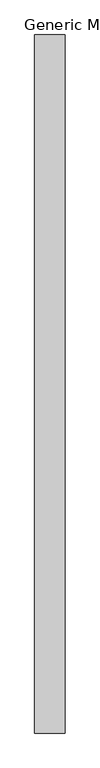
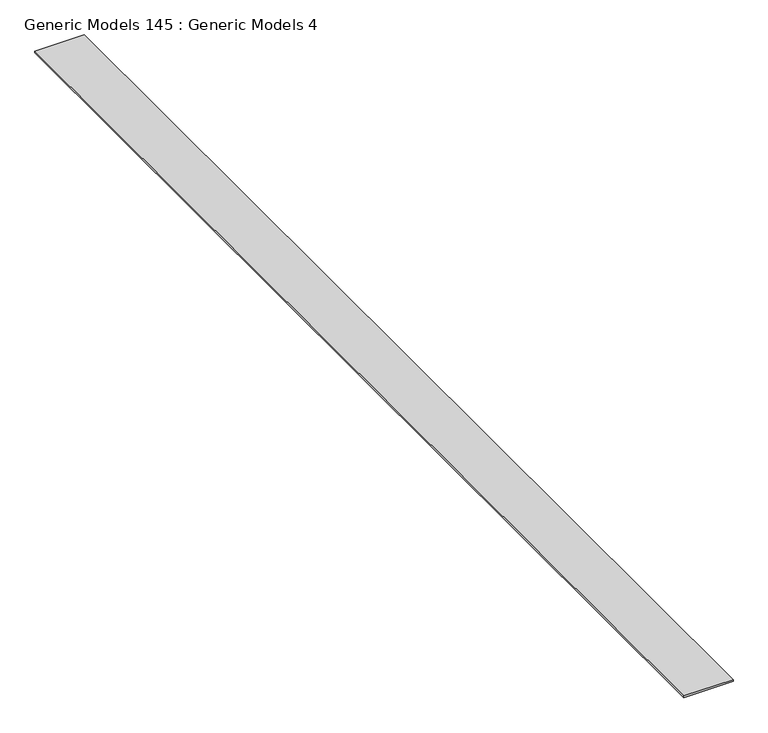
"""IFC4 building model written with IfcOpenShell, lengths in millimetres: proxy geometry, Generic Models 145 : Generic Models 4."""

from ifc_helpers import new_model, si_unit, frame, origin, place, context, project, spatial, polyline, outline, extrude, source, transform, mapped, element, save


def generic_models_145_generic_models_4_5156f356(model_context):
    return source(origin(), model_context, "Body", "SweptSolid", [
        extrude(outline(polyline([(-5950.1236296, -5493.3230338), (-6498.6122941, -5493.3230338), (-6498.6122941, 7054.2769662), (-5950.1236296, 7054.2769662), (-5950.1236296, -5493.3230338)])), frame((0.0, 0.0, 123278.646), z_axis=(0.0, 0.0, 1.0), x_axis=(1.0, 0.0, 0.0)), (0.0, 0.0, 1.0), 19.05),
    ])


if __name__ == "__main__":
    model = new_model("IFC4")
    model_context = context("Model", 3, world=origin())
    ifc_project = project(units=[si_unit("LENGTHUNIT", "METRE", prefix="MILLI")], contexts=[model_context])
    site = spatial("IfcSite", under=ifc_project)
    building = spatial("IfcBuilding", under=site)
    placement = place(None, origin())
    generic_models_145_generic_models_4_shape = generic_models_145_generic_models_4_5156f356(model_context)
    element("IfcBuildingElementProxy", 1, Name="Generic Models 145 : Generic Models 4", ObjectType="Generic Models 145 : Generic Models 4", at=placement, inside=building, context=model_context, shape_type="MappedRepresentation", body=[
        mapped(generic_models_145_generic_models_4_shape, transform((0.0, 0.0, 0.0), x_axis=(1.0, 0.0, 0.0), y_axis=(0.0, 1.0, 0.0), z_axis=(0.0, 0.0, 1.0))),
    ])
    save(model, "model.ifc")

# Revit data of these elements
# Element 1 (IfcBuildingElementProxy, "Generic Models 145 : Generic Models 4")
#   Materials on its faces: "_WOOD FLOORING (SPEC T.B.D.)"
# Materials
#   "_WOOD FLOORING (SPEC T.B.D.)": class "Generic", colour RGB 177 130 114, transparency 0, Cost = 0
